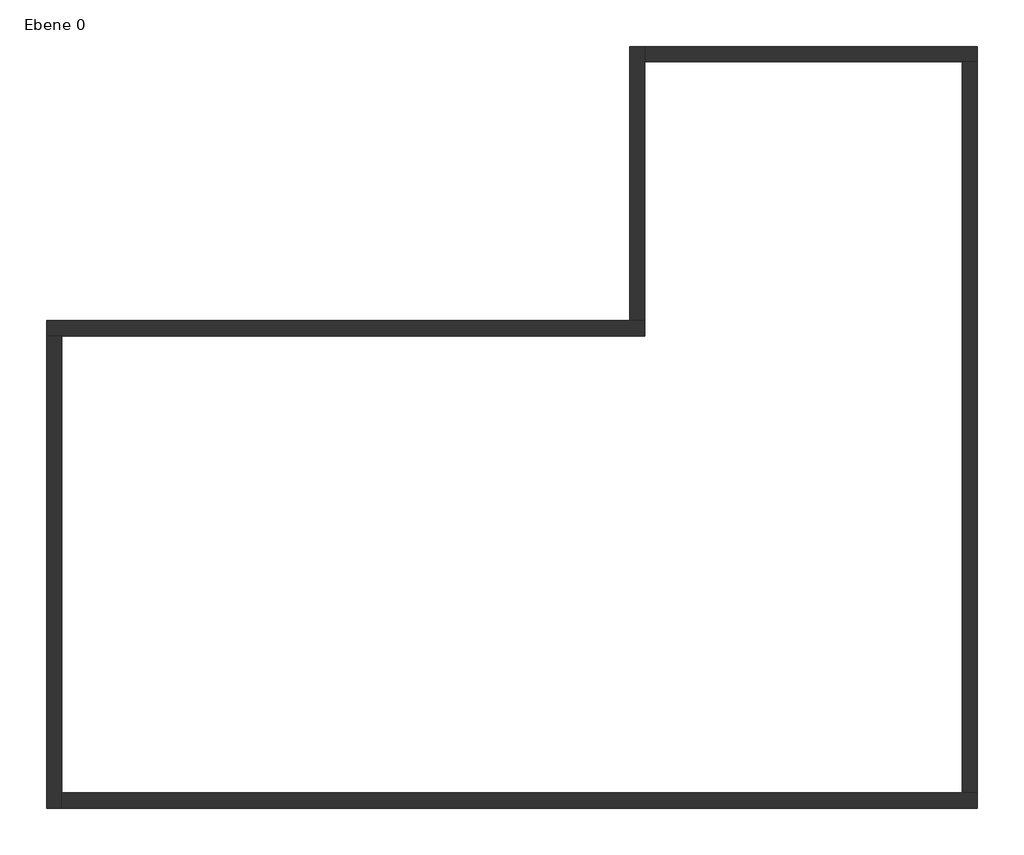
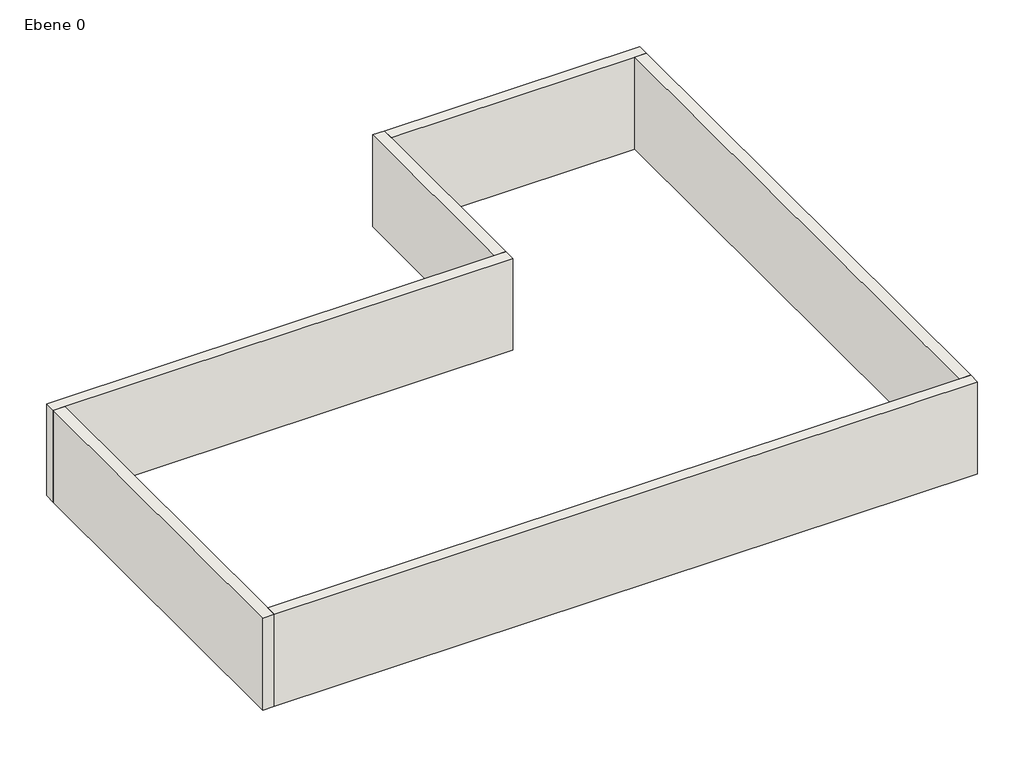
# One storey: 6 walls.
"""IFC4 building model written with IfcOpenShell, lengths in millimetres."""

import ifcopenshell
import ifcopenshell.guid

model = None  # the IFC model being written
_history = None  # IfcOwnerHistory: only IFC2X3 demands one
_inside = {}  # id of a spatial element -> (the spatial element, [elements in it])
_under = {}  # id of a project, library or spatial element -> (it, [spatial elements below it])
_declared = {}  # id of a project -> (the project, [libraries it declares])
_typed = {}  # id of a type object -> (the type object, [elements of that type])
_made_of = {}  # id of a material, layer set ... -> (it, [elements and type objects made of it])


def new_model(schema):
    """Start an empty IFC model of exactly this schema.

    Asked for "IFC4X3", IfcOpenShell would pick the latest addendum, in which some entities
    have other attributes; the version numbers below select the first issue.
    IFC2X3 requires an IfcOwnerHistory on every rooted entity: one is made here for all.
    """
    global model, _history
    if schema == "IFC4X3":
        model = ifcopenshell.file(schema_version=(4, 3, 0, 0))
    else:
        model = ifcopenshell.file(schema=schema)
    _inside.clear()
    _under.clear()
    _declared.clear()
    _typed.clear()
    _made_of.clear()
    _history = None
    if model.schema == "IFC2X3":
        org = make("IfcOrganization", Name="unknown")
        user = make(
            "IfcPersonAndOrganization",
            ThePerson=make("IfcPerson", FamilyName="unknown"),
            TheOrganization=org,
        )
        app = make(
            "IfcApplication",
            ApplicationDeveloper=org,
            Version="unknown",
            ApplicationFullName="unknown",
            ApplicationIdentifier="unknown",
        )
        _history = make(
            "IfcOwnerHistory",
            OwningUser=user,
            OwningApplication=app,
            ChangeAction="ADDED",
            CreationDate=0,
        )
    return model


def make(cls, **values):
    """One entity of the class cls with the attributes given. An attribute that is None is left unset."""
    return model.create_entity(
        cls, **{name: value for name, value in values.items() if value is not None}
    )


def rooted(cls, **values):
    """An entity with a GlobalId (a new one), such as an element, a storey or a relation."""
    return make(cls, GlobalId=ifcopenshell.guid.new(), OwnerHistory=_history, **values)


def si_unit(unit_type, name, prefix=None):
    """IfcSIUnit, for example si_unit("LENGTHUNIT", "METRE", prefix="MILLI")."""
    return make("IfcSIUnit", UnitType=unit_type, Prefix=prefix, Name=name)


def assignment(units):
    """IfcUnitAssignment: the units of a project."""
    return None if units is None else make("IfcUnitAssignment", Units=units)


def point(xyz):
    """IfcCartesianPoint."""
    return None if xyz is None else make("IfcCartesianPoint", Coordinates=xyz)


def direction(xyz):
    """IfcDirection."""
    return None if xyz is None else make("IfcDirection", DirectionRatios=xyz)


def frame(location, z_axis=None, x_axis=None):
    """IfcAxis2Placement3D, a coordinate frame: its origin and axes. An axis left out is left unset."""
    return make(
        "IfcAxis2Placement3D",
        Location=point(location),
        Axis=direction(z_axis),
        RefDirection=direction(x_axis),
    )


def origin():
    """The frame at (0, 0, 0) with its axes left unset."""
    return frame((0.0, 0.0, 0.0))


def origin_with_axes():
    """The frame at (0, 0, 0) with the z axis (0, 0, 1) and the x axis (1, 0, 0) written out."""
    return frame((0.0, 0.0, 0.0), z_axis=(0.0, 0.0, 1.0), x_axis=(1.0, 0.0, 0.0))


def place(relative_to, where):
    """IfcLocalPlacement: puts the frame where relative to a parent placement (None: the world)."""
    return make(
        "IfcLocalPlacement", PlacementRelTo=relative_to, RelativePlacement=where
    )


def context(
    kind, dimensions, precision=None, world=None, true_north=None, identifier=None
):
    """IfcGeometricRepresentationContext, for example the 3D "Model" context."""
    return make(
        "IfcGeometricRepresentationContext",
        ContextIdentifier=identifier,
        ContextType=kind,
        CoordinateSpaceDimension=dimensions,
        Precision=precision,
        WorldCoordinateSystem=world,
        TrueNorth=true_north,
    )


def project(units=None, contexts=None):
    """IfcProject with its units and contexts."""
    return rooted(
        "IfcProject",
        Name="project",
        RepresentationContexts=contexts,
        UnitsInContext=assignment(units),
    )


def spatial(cls, under=None, at=None, **own):
    """A site, building, storey or space (cls), placed at a placement, below another one or the project."""
    s = rooted(cls, ObjectPlacement=at, **own)
    if under is not None:
        _under.setdefault(under.id(), (under, []))[1].append(s)
    return s


def polyline(points):
    """IfcPolyline through the points."""
    return make("IfcPolyline", Points=[point(p) for p in points])


def outline(outer, holes=None, kind="AREA"):
    """IfcArbitraryClosedProfileDef: a profile drawn as a closed curve; with holes, ...WithVoids."""
    if holes is None:
        return make("IfcArbitraryClosedProfileDef", ProfileType=kind, OuterCurve=outer)
    return make(
        "IfcArbitraryProfileDefWithVoids",
        ProfileType=kind,
        OuterCurve=outer,
        InnerCurves=holes,
    )


def extrude(swept, where, along, depth):
    """IfcExtrudedAreaSolid: the profile swept, set in the frame where, extruded along a direction by depth."""
    return make(
        "IfcExtrudedAreaSolid",
        SweptArea=swept,
        Position=where,
        ExtrudedDirection=direction(along),
        Depth=depth,
    )


def faces_of(points, faces, orient=None, outer=None):
    """IfcFace entities. A face is a list of loops; a loop is a list of indices into points, from 0.

    orient and outer hold one flag for each loop. By default every Orientation is true, the
    first loop of a face is its IfcFaceOuterBound and the others are IfcFaceBound.
    """
    made = []
    for i, loops in enumerate(faces):
        bounds = []
        for j, loop in enumerate(loops):
            is_outer = j == 0 if outer is None else outer[i][j]
            bounds.append(
                make(
                    "IfcFaceOuterBound" if is_outer else "IfcFaceBound",
                    Bound=make("IfcPolyLoop", Polygon=[points[k] for k in loop]),
                    Orientation=True if orient is None else orient[i][j],
                )
            )
        made.append(make("IfcFace", Bounds=bounds))
    return made


def faceted_brep(points, faces, orient=None, outer=None, voids=None):
    """IfcFacetedBrep: a solid bounded by flat faces; with voids (closed shells), ...WithVoids."""
    shared = [point(p) for p in points]
    hull = make("IfcClosedShell", CfsFaces=faces_of(shared, faces, orient, outer))
    if voids is None:
        return make("IfcFacetedBrep", Outer=hull)
    return make(
        "IfcFacetedBrepWithVoids",
        Outer=hull,
        Voids=[
            make(cls, CfsFaces=faces_of(shared, fs, o, b)) for cls, fs, o, b in voids
        ],
    )


def shape(context_of_items, identifier, shape_type, items):
    """IfcShapeRepresentation: the items that make up one representation, for example the "Body"."""
    return make(
        "IfcShapeRepresentation",
        ContextOfItems=context_of_items,
        RepresentationIdentifier=identifier,
        RepresentationType=shape_type,
        Items=items,
    )


def made_of(thing, what):
    """Note that an element or type object is made of a material, layer set ...; save() writes the relation."""
    if what is not None:
        _made_of.setdefault(what.id(), (what, []))[1].append(thing)
    return thing


def element(
    cls,
    number,
    at=None,
    inside=None,
    cuts=None,
    type_object=None,
    material=None,
    context=None,
    identifier="Body",
    shape_type=None,
    held_by="IfcProductDefinitionShape",
    body=None,
    shapes=None,
    **own,
):
    """One element of the class cls, such as IfcWall. Its Tag is "e" and its number.

    at: its placement. inside: the storey or other place that contains it. cuts: it is an
    opening in that element (IfcRelVoidsElement). A single representation is given by context,
    identifier, shape_type and body (its items); several are given by shapes. held_by: the class
    of the entity that holds the representations. save() writes the other relations.
    """
    e = rooted(cls, Tag="e%d" % number, ObjectPlacement=at, **own)
    if body is not None:
        shapes = [shape(context, identifier, shape_type, body)]
    if shapes is not None:
        e.Representation = make(held_by, Representations=shapes)
    if inside is not None:
        _inside.setdefault(inside.id(), (inside, []))[1].append(e)
    if cuts is not None:
        rooted(
            "IfcRelVoidsElement", RelatingBuildingElement=cuts, RelatedOpeningElement=e
        )
    if type_object is not None:
        _typed.setdefault(type_object.id(), (type_object, []))[1].append(e)
    return made_of(e, material)


def aggregate(whole, parts):
    """IfcRelAggregates: a whole, such as a stair, and the parts it consists of."""
    return rooted("IfcRelAggregates", RelatingObject=whole, RelatedObjects=parts)


def save(model, path):
    """Write the relations noted so far, then the file.

    IfcRelAggregates (storeys below a building ...), IfcRelContainedInSpatialStructure (elements
    in a storey), IfcRelDefinesByType, IfcRelAssociatesMaterial and IfcRelDeclares: one each for
    every whole, place, type object, material and project.
    """
    for whole, parts in _under.values():
        aggregate(whole, parts)
    for where, things in _inside.values():
        rooted(
            "IfcRelContainedInSpatialStructure",
            RelatedElements=things,
            RelatingStructure=where,
        )
    for kind, things in _typed.values():
        rooted("IfcRelDefinesByType", RelatedObjects=things, RelatingType=kind)
    for what, things in _made_of.values():
        rooted("IfcRelAssociatesMaterial", RelatedObjects=things, RelatingMaterial=what)
    for by, libraries in _declared.values():
        rooted("IfcRelDeclares", RelatingContext=by, RelatedDefinitions=libraries)
    model.write(path)


model = new_model("IFC4")

# Units and contexts
model_context = context("Model", 3, world=origin())
ifc_project = project(units=[si_unit("LENGTHUNIT", "METRE", prefix="MILLI")], contexts=[model_context])

# Site, building, storey
site = spatial("IfcSite", under=ifc_project)
building = spatial("IfcBuilding", under=site)
storey = spatial("IfcBuildingStorey", under=building, Name="Ebene 0", Elevation=0.0)

# Walls
placement = place(None, origin())
element("IfcWall", 1, ObjectType="MW 24.0 WD 12.0", at=placement, inside=storey, context=model_context, shape_type="Brep", body=[
    faceted_brep([(-13369.6797169, 6985.6067473, 0.0), (-13009.6797169, 6985.6067473, 0.0), (810.3202831, 6985.6067473, 0.0), (810.3202831, 6985.6067473, 3000.0), (-13009.6797169, 6985.6067473, 3000.0), (-13369.6797169, 6985.6067473, 3000.0), (-13369.6797169, 7345.6067473, 0.0), (-13369.6797169, 7345.6067473, 3000.0), (450.3202831, 7345.6067473, 3000.0), (810.3202831, 7345.6067473, 3000.0), (810.3202831, 7345.6067473, 0.0), (450.3202831, 7345.6067473, 0.0)], [[[0, 1, 2, 3, 4, 5]], [[6, 7, 8, 9, 10, 11]], [[2, 1, 0, 6, 11, 10]], [[5, 4, 3, 9, 8, 7]], [[0, 5, 7, 6]], [[3, 2, 10, 9]]]),
])
element("IfcWall", 2, ObjectType="MW 24.0 WD 12.0", at=placement, inside=storey, context=model_context, shape_type="Brep", body=[
    faceted_brep([(-13009.6797169, -4214.3932527, 0.0), (-13009.6797169, -3854.3932527, 0.0), (-13009.6797169, 6985.6067473, 0.0), (-13009.6797169, 6985.6067473, 3000.0), (-13009.6797169, -3854.3932527, 3000.0), (-13009.6797169, -4214.3932527, 3000.0), (-13369.6797169, -4214.3932527, 0.0), (-13369.6797169, -4214.3932527, 3000.0), (-13369.6797169, 6985.6067473, 3000.0), (-13369.6797169, 6985.6067473, 0.0)], [[[0, 1, 2, 3, 4, 5]], [[6, 7, 8, 9]], [[2, 1, 0, 6, 9]], [[5, 4, 3, 8, 7]], [[0, 5, 7, 6]], [[3, 2, 9, 8]]]),
])
element("IfcWall", 3, ObjectType="MW 24.0 WD 12.0", at=placement, inside=storey, context=model_context, shape_type="Brep", body=[
    faceted_brep([(8690.3202831, -3854.3932527, 0.0), (8330.3202831, -3854.3932527, 0.0), (-13009.6797169, -3854.3932527, 0.0), (-13009.6797169, -3854.3932527, 3000.0), (8330.3202831, -3854.3932527, 3000.0), (8690.3202831, -3854.3932527, 3000.0), (8690.3202831, -4214.3932527, 0.0), (8690.3202831, -4214.3932527, 3000.0), (-13009.6797169, -4214.3932527, 3000.0), (-13009.6797169, -4214.3932527, 0.0)], [[[0, 1, 2, 3, 4, 5]], [[6, 7, 8, 9]], [[2, 1, 0, 6, 9]], [[5, 4, 3, 8, 7]], [[0, 5, 7, 6]], [[3, 2, 9, 8]]]),
])
element("IfcWall", 4, ObjectType="MW 24.0 WD 12.0", at=placement, inside=storey, context=model_context, shape_type="SweptSolid", body=[
    extrude(outline(polyline([(8330.3202831, -3854.3932527), (8330.3202831, 13485.6067473), (8690.3202831, 13485.6067473), (8690.3202831, -3854.3932527), (8330.3202831, -3854.3932527)])), origin_with_axes(), (0.0, 0.0, 1.0), 3000.0),
])
element("IfcWall", 5, ObjectType="MW 24.0 WD 12.0", at=placement, inside=storey, context=model_context, shape_type="Brep", body=[
    faceted_brep([(810.3202831, 7345.6067473, 0.0), (810.3202831, 13485.6067473, 0.0), (810.3202831, 13845.6067473, 0.0), (810.3202831, 13845.6067473, 3000.0), (810.3202831, 13485.6067473, 3000.0), (810.3202831, 7345.6067473, 3000.0), (450.3202831, 7345.6067473, 0.0), (450.3202831, 7345.6067473, 3000.0), (450.3202831, 13845.6067473, 3000.0), (450.3202831, 13845.6067473, 0.0)], [[[0, 1, 2, 3, 4, 5]], [[6, 7, 8, 9]], [[2, 1, 0, 6, 9]], [[5, 4, 3, 8, 7]], [[3, 2, 9, 8]], [[0, 5, 7, 6]]]),
])
element("IfcWall", 6, ObjectType="MW 24.0 WD 12.0", at=placement, inside=storey, context=model_context, shape_type="Brep", body=[
    faceted_brep([(810.3202831, 13485.6067473, 0.0), (8330.3202831, 13485.6067473, 0.0), (8690.3202831, 13485.6067473, 0.0), (8690.3202831, 13485.6067473, 3000.0), (8330.3202831, 13485.6067473, 3000.0), (810.3202831, 13485.6067473, 3000.0), (810.3202831, 13845.6067473, 0.0), (810.3202831, 13845.6067473, 3000.0), (8690.3202831, 13845.6067473, 3000.0), (8690.3202831, 13845.6067473, 0.0)], [[[0, 1, 2, 3, 4, 5]], [[6, 7, 8, 9]], [[2, 1, 0, 6, 9]], [[5, 4, 3, 8, 7]], [[0, 5, 7, 6]], [[3, 2, 9, 8]]]),
])

save(model, "model.ifc")

# Revit data of these elements
# Project information
#   Projektausgabedatum = "Projekt Datum"
#   Projektstatus = "Projektstatus"
#   Kundenname = "Bauherr"
#   Projektadresse = "Projektadresse"
#   Projektname = "Projektname"
#   Projektnummer = "Projektnummer"
#   Verfasser Firma 1 = "Firma 1"
#   Verfasser Firma 2 = "Firma 2"
#   Verfasser PLZ Ort = "PLZ Ort"
#   Verfasser Strasse = "Strasse"
#   Verfasser Telefon = "Telefon"
#   Verfasser Telefax = "Telefax"
#   Verfasser eMail = "E-Mail"
# Type "MW 24.0 WD 12.0"
#   Type Comments = "Mehrschaliges Mauerwerk"
#   Description = "Mauerwerk 24.0 cm, Wärmedämmung 12.0 cm"
#   Width = 0.360 m
#   Layers, outside or top first: 0.120 m "Wärmedämmung - Hart" (function 3); 0.240 m "Mauerwerk - Ziegel, verputzt" (function 1)
# Element 1 (IfcWall, "MW 24.0 WD 12.0")
#   Top Offset = 0.000 m
#   Base Offset = 0.000 m
#   wall height = 3.000 m
#   Phase Created = Phase 1
#   Base Constraint = Ebene 0
#   Top Constraint = Ebene 1
#   Materials on its faces: "Mauerwerk - Ziegel, verputzt", "Wärmedämmung - Hart", "Standard - Wand"
# Elements 2, 3, 5, 6 (IfcWall, "MW 24.0 WD 12.0")
#   Top Offset = 0.000 m
#   Base Offset = 0.000 m
#   wall height = 3.000 m
#   Phase Created = Phase 1
#   Base Constraint = Ebene 0
#   Top Constraint = Ebene 1
#   Materials on its faces: "Standard - Wand", "Wärmedämmung - Hart", "Mauerwerk - Ziegel, verputzt"
# Element 4 (IfcWall, "MW 24.0 WD 12.0")
#   Top Offset = 0.000 m
#   Base Offset = 0.000 m
#   wall height = 3.000 m
#   Phase Created = Phase 1
#   Base Constraint = Ebene 0
#   Top Constraint = Ebene 1
#   Materials on its faces: "Standard - Wand", "Mauerwerk - Ziegel, verputzt", "Wärmedämmung - Hart"
# Materials
#   "Wärmedämmung - Hart": class "Putz", colour RGB 255 255 255, transparency 0, Description = "Äußere Oberfläche"
#   "Mauerwerk - Ziegel, verputzt": class "Putz", colour RGB 247 247 247, transparency 0, Cost = 0
#   "Standard - Wand": class "Putz", colour RGB 128 128 128, transparency 0, Description = "Äußere Oberfläche"
